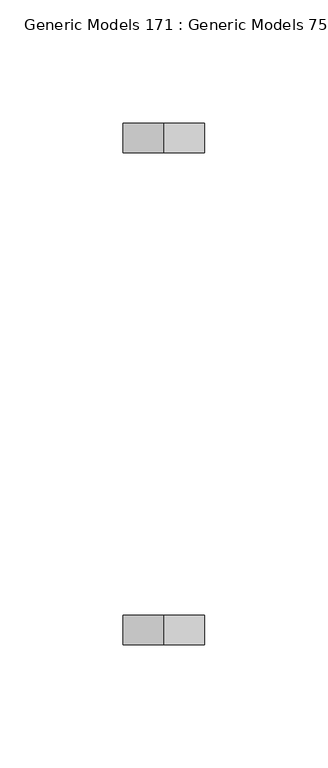
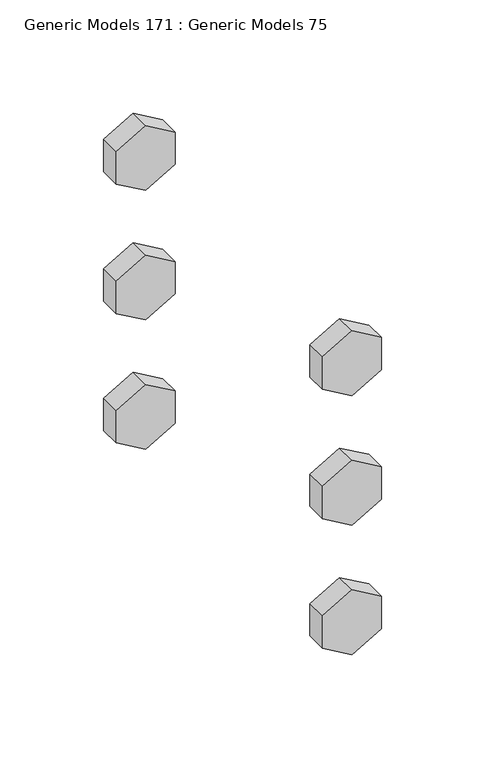
"""IFC4 building model written with IfcOpenShell, lengths in millimetres: proxy geometry, Generic Models 171 : Generic Models 75."""

from ifc_helpers import new_model, si_unit, frame, origin, place, context, project, spatial, polyline, outline, extrude, source, transform, mapped, element, save


def generic_models_171_generic_models_75_5ffa0860(model_context):
    return source(origin(), model_context, "Body", "SweptSolid", [
        extrude(outline(polyline([(269043.15, 31735.8680692), (269033.625, 31752.3658532), (269043.15, 31768.8636371), (269062.2, 31768.8636371), (269071.725, 31752.3658532), (269062.2, 31735.8680692), (269043.15, 31735.8680692)])), frame((0.0, 30868.0031612, 0.0), z_axis=(0.0, 1.0, 0.0), x_axis=(0.0, 0.0, 1.0)), (0.0, 0.0, 1.0), 11.90625),
        extrude(outline(polyline([(268966.95, 31735.8680692), (268957.425, 31752.3658532), (268966.95, 31768.8636371), (268986.0, 31768.8636371), (268995.525, 31752.3658532), (268986.0, 31735.8680692), (268966.95, 31735.8680692)])), frame((0.0, 30868.0031612, 0.0), z_axis=(0.0, 1.0, 0.0), x_axis=(0.0, 0.0, 1.0)), (0.0, 0.0, 1.0), 11.90625),
        extrude(outline(polyline([(268890.75, 31735.8680692), (268881.225, 31752.3658532), (268890.75, 31768.8636371), (268909.8, 31768.8636371), (268919.325, 31752.3658532), (268909.8, 31735.8680692), (268890.75, 31735.8680692)])), frame((0.0, 30868.0031612, 0.0), z_axis=(0.0, 1.0, 0.0), x_axis=(0.0, 0.0, 1.0)), (0.0, 0.0, 1.0), 11.90625),
        extrude(outline(polyline([(269043.15, 31735.8680692), (269033.625, 31752.3658532), (269043.15, 31768.8636371), (269062.2, 31768.8636371), (269071.725, 31752.3658532), (269062.2, 31735.8680692), (269043.15, 31735.8680692)])), frame((0.0, 30668.7719112, 0.0), z_axis=(0.0, 1.0, 0.0), x_axis=(0.0, 0.0, 1.0)), (0.0, 0.0, 1.0), 11.90625),
        extrude(outline(polyline([(268966.95, 31735.8680692), (268957.425, 31752.3658532), (268966.95, 31768.8636371), (268986.0, 31768.8636371), (268995.525, 31752.3658532), (268986.0, 31735.8680692), (268966.95, 31735.8680692)])), frame((0.0, 30668.7719112, 0.0), z_axis=(0.0, 1.0, 0.0), x_axis=(0.0, 0.0, 1.0)), (0.0, 0.0, 1.0), 11.90625),
        extrude(outline(polyline([(268890.75, 31735.8680692), (268881.225, 31752.3658532), (268890.75, 31768.8636371), (268909.8, 31768.8636371), (268919.325, 31752.3658532), (268909.8, 31735.8680692), (268890.75, 31735.8680692)])), frame((0.0, 30668.7719112, 0.0), z_axis=(0.0, 1.0, 0.0), x_axis=(0.0, 0.0, 1.0)), (0.0, 0.0, 1.0), 11.90625),
    ])


if __name__ == "__main__":
    model = new_model("IFC4")
    model_context = context("Model", 3, world=origin())
    ifc_project = project(units=[si_unit("LENGTHUNIT", "METRE", prefix="MILLI")], contexts=[model_context])
    site = spatial("IfcSite", under=ifc_project)
    building = spatial("IfcBuilding", under=site)
    placement = place(None, origin())
    generic_models_171_generic_models_75_shape = generic_models_171_generic_models_75_5ffa0860(model_context)
    element("IfcBuildingElementProxy", 1, Name="Generic Models 171 : Generic Models 75", ObjectType="Generic Models 171 : Generic Models 75", at=placement, inside=building, context=model_context, shape_type="MappedRepresentation", body=[
        mapped(generic_models_171_generic_models_75_shape, transform((0.0, 0.0, 0.0), x_axis=(1.0, 0.0, 0.0), y_axis=(0.0, 1.0, 0.0), z_axis=(0.0, 0.0, 1.0))),
    ])
    save(model, "model.ifc")
